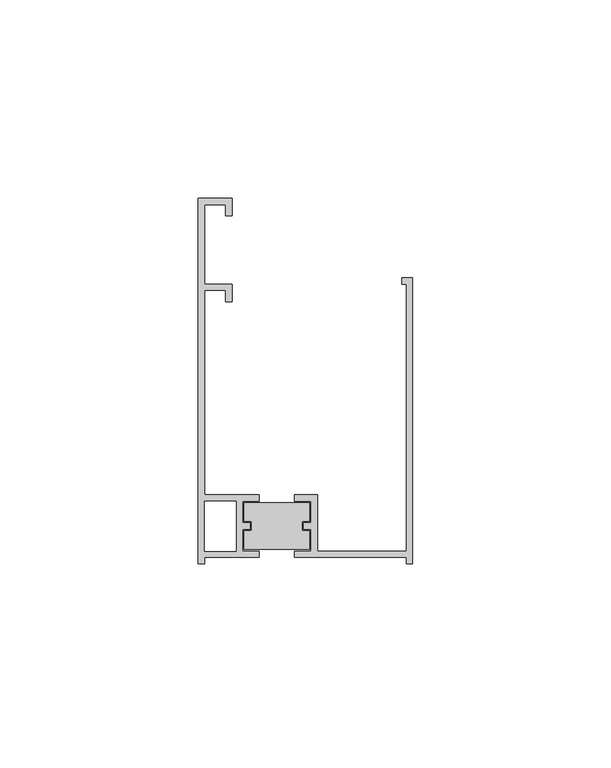
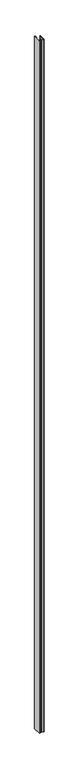
"""IFC4 building model written with IfcOpenShell, lengths in millimetres: proxy geometry, Generic Models 2:Generic Models 2:310765:Generic Models 2:310765 : Generic Models 2:Generic Models 2:310765:60 : Generic Models 2:Generic Models 2:310765:Generic Models 2:310765 : Generic Models 2:Generic Models 2:310765:300385."""

from ifc_helpers import new_model, si_unit, frame, origin, place, context, project, spatial, polyline, outline, extrude, source, transform, mapped, element, save


def generic_models_8a739291(model_context):
    return source(origin(), model_context, "Body", "SweptSolid", [
        extrude(outline(polyline([(667633.5969099, -465596.2158643), (667633.5969099, -465600.9133629), (667631.6714944, -465600.9133629), (667631.6714944, -465603.2946129), (667633.5969099, -465603.2946129), (667633.5969099, -465607.9921116), (667617.0446537, -465607.9921116), (667617.0446537, -465603.2946129), (667618.9700691, -465603.2946129), (667618.9700691, -465600.9133629), (667617.0446537, -465600.9133629), (667617.0446537, -465596.2158643), (667633.5969099, -465596.2158643)])), frame((0.0, 0.0, 118.1435632), z_axis=(0.0, 0.0, 1.0), x_axis=(1.0, 0.0, 0.0)), (0.0, 0.0, 1.0), 8437.624436),
        extrude(outline(polyline([(667613.9760152, -465519.5639866), (667613.9760152, -465523.9513131), (667612.3885152, -465523.9513131), (667612.3885152, -465521.1514866), (667607.1171437, -465521.1514866), (667607.1171437, -465541.1514866), (667613.9760152, -465541.1514866), (667613.9760152, -465545.5388131), (667612.3885152, -465545.5388131), (667612.3885152, -465542.7389866), (667607.1171437, -465542.7389866), (667607.1171437, -465594.2314893), (667620.8149662, -465594.2314893), (667620.8149662, -465595.8189893), (667616.6477787, -465595.8189893), (667616.6477787, -465601.3102379), (667618.5731941, -465601.3102379), (667618.5731941, -465602.8977379), (667616.6477787, -465602.8977379), (667616.6477787, -465608.3889866), (667620.8149662, -465608.3889866), (667620.8149662, -465609.9764866), (667607.1171437, -465609.9764866), (667607.1171437, -465611.5639866), (667605.5296437, -465611.5639866), (667605.5296437, -465519.5639866), (667613.9760152, -465519.5639866)]), holes=[polyline([(667607.1171437, -465595.8189893), (667607.1171437, -465608.3889866), (667615.0602787, -465608.3889866), (667615.0602787, -465595.8189893), (667607.1171437, -465595.8189893)])]), frame((0.0, 0.0, 118.1435632), z_axis=(0.0, 0.0, 1.0), x_axis=(1.0, 0.0, 0.0)), (0.0, 0.0, 1.0), 8437.624436),
        extrude(outline(polyline([(667657.9421437, -465611.5639866), (667657.9421437, -465609.9764866), (667629.8265974, -465609.9764866), (667629.8265974, -465608.3889866), (667633.9937849, -465608.3889866), (667633.9937849, -465602.8977379), (667632.0683694, -465602.8977379), (667632.0683694, -465601.3102379), (667633.9937849, -465601.3102379), (667633.9937849, -465595.8189893), (667629.8265974, -465595.8189893), (667629.8265974, -465594.2314893), (667635.5812849, -465594.2314893), (667635.5812849, -465608.3889866), (667657.9421437, -465608.3889866), (667657.9421437, -465541.1514866), (667656.8145537, -465541.1514866), (667656.8145537, -465539.5639866), (667659.5296437, -465539.5639866), (667659.5296437, -465611.5639866), (667657.9421437, -465611.5639866)])), frame((0.0, 0.0, 118.1435632), z_axis=(0.0, 0.0, 1.0), x_axis=(1.0, 0.0, 0.0)), (0.0, 0.0, 1.0), 8437.624436),
    ])


if __name__ == "__main__":
    model = new_model("IFC4")
    model_context = context("Model", 3, world=origin())
    ifc_project = project(units=[si_unit("LENGTHUNIT", "METRE", prefix="MILLI")], contexts=[model_context])
    site = spatial("IfcSite", under=ifc_project)
    building = spatial("IfcBuilding", under=site)
    placement = place(None, origin())
    generic_models_shape = generic_models_8a739291(model_context)
    element("IfcBuildingElementProxy", 1, Name="Generic Models 2:Generic Models 2:310765:Generic Models 2:310765 : Generic Models 2:Generic Models 2:310765:60 : Generic Models 2:Generic Models 2:310765:Generic Models 2:310765 : Generic Models 2:Generic Models 2:310765:300385", ObjectType="Generic Models 2:Generic Models 2:310765:Generic Models 2:310765 : Generic Models 2:Generic Models 2:310765:60 : Generic Models 2:Generic Models 2:310765:Generic Models 2:310765 : Generic Models 2:Generic Models 2:310765:300385", at=placement, inside=building, context=model_context, shape_type="MappedRepresentation", body=[
        mapped(generic_models_shape, transform((0.0, 0.0, 0.0), x_axis=(1.0, 0.0, 0.0), y_axis=(0.0, 1.0, 0.0), z_axis=(0.0, 0.0, 1.0))),
    ])
    save(model, "model.ifc")

# Revit data of these elements
# Type "Generic Models 2:Generic Models 2:310765:Generic Models 2:310765 : Generic Models 2:Generic Models 2:310765:60 : Generic Models 2:Generic Models 2:310765:Generic Models 2:310765 : Generic Models 2:Generic Models 2:310765:300385"
#   NameOverride = "Generic Models 2:Generic Models 2:310765:Generic Models 2:310765 : Generic Models 2:Generic Models 2:310765:300385"
#   ObjectTypeOverride = "Generic Models 2:310765 : Generic Models 2:Generic Models 2:310765"
#   Reference = "Generic Models 2"
#   Tag = "300385"
# Element 1 (IfcBuildingElementProxy, "Generic Models 2:Generic Models 2:310765:Generic Models 2:310765 : Generic Models 2:Generic Models 2:310765:60 : Generic Models 2:Generic Models 2:310765:Generic Models 2:310765 : Generic Models 2:Generic Models 2:310765:300385")
#   Materials on its faces: "THERMAL BROKEN ALUMINUM STOREFRONT FOR POLYCARBONATE"
# Materials
#   "THERMAL BROKEN ALUMINUM STOREFRONT FOR POLYCARBONATE": class "Unassigned", colour RGB 244 244 244, transparency 0, Keynote = "M07611300.01", Cost = 0
